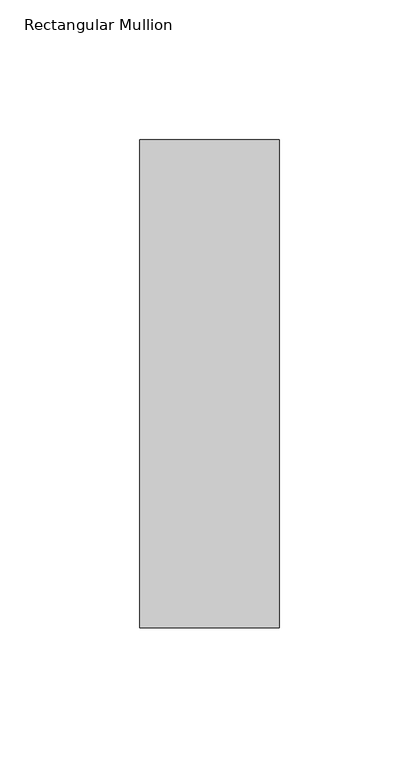
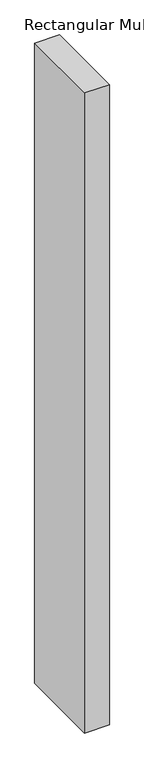
"""IFC4 building model written with IfcOpenShell, lengths in millimetres: member geometry, Rectangular Mullion : WWm-50x175-50mmOffset."""

from ifc_helpers import new_model, si_unit, frame, origin, place, context, project, spatial, polyline, outline, extrude, source, transform, mapped, element, save


def rectangular_mullion_bdb9034a(model_context):
    return source(origin(), model_context, "Body", "SweptSolid", [
        extrude(outline(polyline([(0.0, 87.5), (0.0, -87.5), (-50.0, -87.5), (-50.0, 87.5), (0.0, 87.5)])), frame((0.0, 0.0, -1370.0), z_axis=(0.0, 0.0, 1.0), x_axis=(1.0, 0.0, 0.0)), (0.0, 0.0, 1.0), 1370.0),
    ])


if __name__ == "__main__":
    model = new_model("IFC4")
    model_context = context("Model", 3, world=origin())
    ifc_project = project(units=[si_unit("LENGTHUNIT", "METRE", prefix="MILLI")], contexts=[model_context])
    site = spatial("IfcSite", under=ifc_project)
    building = spatial("IfcBuilding", under=site)
    placement = place(None, origin())
    rectangular_mullion_shape = rectangular_mullion_bdb9034a(model_context)
    element("IfcMember", 1, ObjectType="Rectangular Mullion : WWm-50x175-50mmOffset", at=placement, inside=building, context=model_context, shape_type="MappedRepresentation", body=[
        mapped(rectangular_mullion_shape, transform((0.0, 0.0, 0.0), x_axis=(1.0, 0.0, 0.0), y_axis=(0.0, 1.0, 0.0), z_axis=(0.0, 0.0, 1.0))),
    ])
    save(model, "model.ifc")

# Revit data of these elements
# Type "Rectangular Mullion : WWm-50x175-50mmOffset"
#   built-in parameter 1007304 = 0.574147 (stored number, unit not read)
#   built-in parameter 1007301 = 0.082021 (stored number, unit not read)
#   built-in parameter 1007300 = 0.082021 (stored number, unit not read)
# Element 1 (IfcMember, "Rectangular Mullion : WWm-50x175-50mmOffset")
#   Materials on its faces: "WW-EC-RGB-Mullion"
# Materials
#   "WW-EC-RGB-Mullion": class "Generic", colour RGB 255 255 255, transparency 0, Comments = "If region requests black mullions, switch asset color to RGB 25-25-25", Description = "Generic Color", Cost = 0
